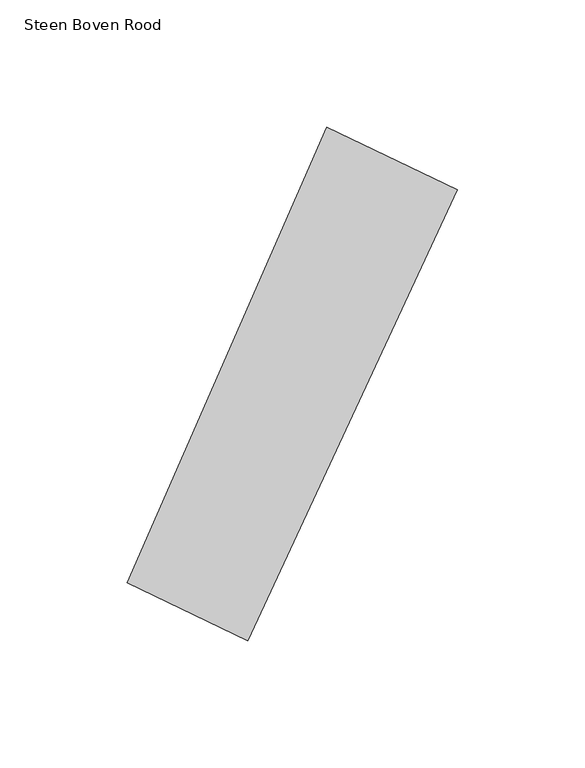
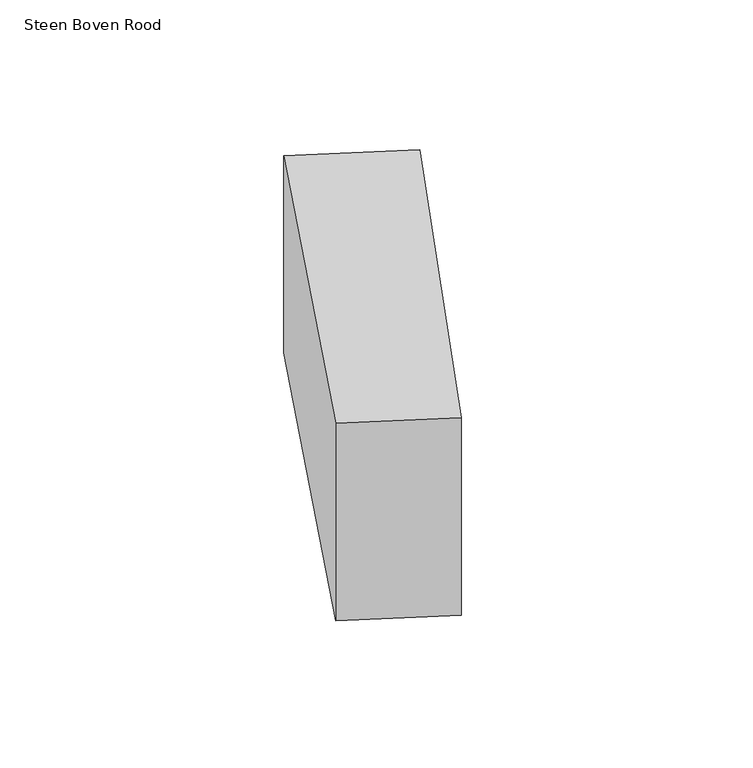
"""IFC4 building model written with IfcOpenShell, lengths in millimetres: proxy geometry, 00_GMA_steen_versie_4 : Steen Boven Rood."""

from ifc_helpers import new_model, si_unit, origin, origin_with_axes, place, context, project, spatial, polyline, outline, extrude, source, transform, mapped, element, save


def steen_boven_rood_4ba1d161(model_context):
    return source(origin(), model_context, "Body", "SweptSolid", [
        extrude(outline(polyline([(143.1721103, 161.4518746), (61.0184626, -15.4115478), (13.8026697, 7.1591713), (92.0476097, 185.8935716), (143.1721103, 161.4518746)])), origin_with_axes(), (0.0, 0.0, 1.0), 100.0),
    ])


if __name__ == "__main__":
    model = new_model("IFC4")
    model_context = context("Model", 3, world=origin())
    ifc_project = project(units=[si_unit("LENGTHUNIT", "METRE", prefix="MILLI")], contexts=[model_context])
    site = spatial("IfcSite", under=ifc_project)
    building = spatial("IfcBuilding", under=site)
    placement = place(None, origin())
    steen_boven_rood_shape = steen_boven_rood_4ba1d161(model_context)
    element("IfcBuildingElementProxy", 1, Name="00_GMA_steen_versie_4 : Steen Boven Rood", ObjectType="00_GMA_steen_versie_4 : Steen Boven Rood", at=placement, inside=building, context=model_context, shape_type="MappedRepresentation", body=[
        mapped(steen_boven_rood_shape, transform((0.0, 0.0, 0.0), x_axis=(1.0, 0.0, 0.0), y_axis=(0.0, 1.0, 0.0), z_axis=(0.0, 0.0, 1.0))),
    ])
    save(model, "model.ifc")

# Revit data of these elements
# Type "00_GMA_steen_versie_4 : Steen Boven Rood"
#   StootVoegHalfBoven [instance default] = 5 mm
#   StootVoegHalf [instance default] = 5 mm
#   StootVoegBreedteOnder = 10 mm
#   StootVoegBreedteBoven = 10 mm
#   Steendikte = 100 mm
#   LintVoegOnderHalf = 5 mm
#   LintVoegOnder = 10 mm
#   LintVoegBovenHalf = 0 mm
#   LintVoegBoven = 0 mm
#   materiaal = 21_steen_rood
#   MateriaalVoeg = none
#   Default Elevation = 0
# Element 1 (IfcBuildingElementProxy, "00_GMA_steen_versie_4 : Steen Boven Rood")
#   Materials on its faces: "21_steen_rood"
# Materials
#   "21_steen_rood": class "Unassigned", colour RGB 213 111 43, transparency 0, Cost = 0
